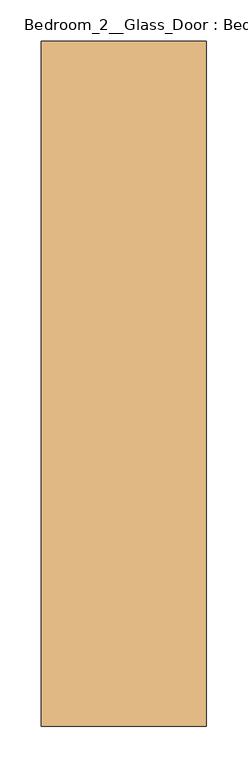
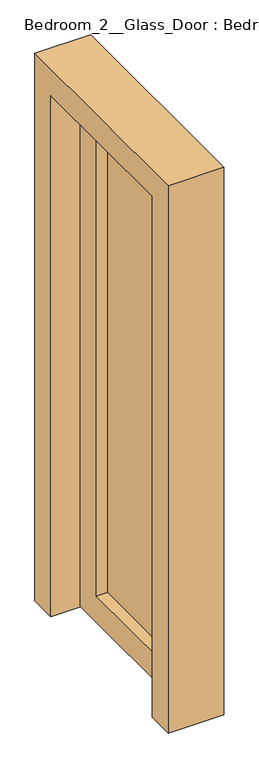
"""IFC4 building model written with IfcOpenShell, lengths in millimetres: door geometry, Bedroom_2__Glass_Door : Bedroom_2__Glass_Door."""

import ifcopenshell
import ifcopenshell.guid

model = None  # the IFC model being written
_history = None  # IfcOwnerHistory: only IFC2X3 demands one
_inside = {}  # id of a spatial element -> (the spatial element, [elements in it])
_under = {}  # id of a project, library or spatial element -> (it, [spatial elements below it])
_declared = {}  # id of a project -> (the project, [libraries it declares])
_typed = {}  # id of a type object -> (the type object, [elements of that type])
_made_of = {}  # id of a material, layer set ... -> (it, [elements and type objects made of it])


def new_model(schema):
    """Start an empty IFC model of exactly this schema.

    Asked for "IFC4X3", IfcOpenShell would pick the latest addendum, in which some entities
    have other attributes; the version numbers below select the first issue.
    IFC2X3 requires an IfcOwnerHistory on every rooted entity: one is made here for all.
    """
    global model, _history
    if schema == "IFC4X3":
        model = ifcopenshell.file(schema_version=(4, 3, 0, 0))
    else:
        model = ifcopenshell.file(schema=schema)
    _inside.clear()
    _under.clear()
    _declared.clear()
    _typed.clear()
    _made_of.clear()
    _history = None
    if model.schema == "IFC2X3":
        org = make("IfcOrganization", Name="unknown")
        user = make(
            "IfcPersonAndOrganization",
            ThePerson=make("IfcPerson", FamilyName="unknown"),
            TheOrganization=org,
        )
        app = make(
            "IfcApplication",
            ApplicationDeveloper=org,
            Version="unknown",
            ApplicationFullName="unknown",
            ApplicationIdentifier="unknown",
        )
        _history = make(
            "IfcOwnerHistory",
            OwningUser=user,
            OwningApplication=app,
            ChangeAction="ADDED",
            CreationDate=0,
        )
    return model


def make(cls, **values):
    """One entity of the class cls with the attributes given. An attribute that is None is left unset."""
    return model.create_entity(
        cls, **{name: value for name, value in values.items() if value is not None}
    )


def rooted(cls, **values):
    """An entity with a GlobalId (a new one), such as an element, a storey or a relation."""
    return make(cls, GlobalId=ifcopenshell.guid.new(), OwnerHistory=_history, **values)


def si_unit(unit_type, name, prefix=None):
    """IfcSIUnit, for example si_unit("LENGTHUNIT", "METRE", prefix="MILLI")."""
    return make("IfcSIUnit", UnitType=unit_type, Prefix=prefix, Name=name)


def assignment(units):
    """IfcUnitAssignment: the units of a project."""
    return None if units is None else make("IfcUnitAssignment", Units=units)


def point(xyz):
    """IfcCartesianPoint."""
    return None if xyz is None else make("IfcCartesianPoint", Coordinates=xyz)


def direction(xyz):
    """IfcDirection."""
    return None if xyz is None else make("IfcDirection", DirectionRatios=xyz)


def frame(location, z_axis=None, x_axis=None):
    """IfcAxis2Placement3D, a coordinate frame: its origin and axes. An axis left out is left unset."""
    return make(
        "IfcAxis2Placement3D",
        Location=point(location),
        Axis=direction(z_axis),
        RefDirection=direction(x_axis),
    )


def origin():
    """The frame at (0, 0, 0) with its axes left unset."""
    return frame((0.0, 0.0, 0.0))


def place(relative_to, where):
    """IfcLocalPlacement: puts the frame where relative to a parent placement (None: the world)."""
    return make(
        "IfcLocalPlacement", PlacementRelTo=relative_to, RelativePlacement=where
    )


def context(
    kind, dimensions, precision=None, world=None, true_north=None, identifier=None
):
    """IfcGeometricRepresentationContext, for example the 3D "Model" context."""
    return make(
        "IfcGeometricRepresentationContext",
        ContextIdentifier=identifier,
        ContextType=kind,
        CoordinateSpaceDimension=dimensions,
        Precision=precision,
        WorldCoordinateSystem=world,
        TrueNorth=true_north,
    )


def project(units=None, contexts=None):
    """IfcProject with its units and contexts."""
    return rooted(
        "IfcProject",
        Name="project",
        RepresentationContexts=contexts,
        UnitsInContext=assignment(units),
    )


def spatial(cls, under=None, at=None, **own):
    """A site, building, storey or space (cls), placed at a placement, below another one or the project."""
    s = rooted(cls, ObjectPlacement=at, **own)
    if under is not None:
        _under.setdefault(under.id(), (under, []))[1].append(s)
    return s


def polyline(points):
    """IfcPolyline through the points."""
    return make("IfcPolyline", Points=[point(p) for p in points])


def outline(outer, holes=None, kind="AREA"):
    """IfcArbitraryClosedProfileDef: a profile drawn as a closed curve; with holes, ...WithVoids."""
    if holes is None:
        return make("IfcArbitraryClosedProfileDef", ProfileType=kind, OuterCurve=outer)
    return make(
        "IfcArbitraryProfileDefWithVoids",
        ProfileType=kind,
        OuterCurve=outer,
        InnerCurves=holes,
    )


def extrude(swept, where, along, depth):
    """IfcExtrudedAreaSolid: the profile swept, set in the frame where, extruded along a direction by depth."""
    return make(
        "IfcExtrudedAreaSolid",
        SweptArea=swept,
        Position=where,
        ExtrudedDirection=direction(along),
        Depth=depth,
    )


def shape(context_of_items, identifier, shape_type, items):
    """IfcShapeRepresentation: the items that make up one representation, for example the "Body"."""
    return make(
        "IfcShapeRepresentation",
        ContextOfItems=context_of_items,
        RepresentationIdentifier=identifier,
        RepresentationType=shape_type,
        Items=items,
    )


def source(mapping_origin, context_of_items, identifier, shape_type, items):
    """IfcRepresentationMap: a shape defined once, which mapped items show again and again."""
    return make(
        "IfcRepresentationMap",
        MappingOrigin=mapping_origin,
        MappedRepresentation=shape(context_of_items, identifier, shape_type, items),
    )


def transform(
    local_origin,
    x_axis=None,
    y_axis=None,
    z_axis=None,
    scale=None,
    scale2=None,
    scale3=None,
    uniform=True,
):
    """IfcCartesianTransformationOperator3D, or its non-uniform kind. x_axis, y_axis, z_axis: its Axis1, 2, 3."""
    if uniform:
        return make(
            "IfcCartesianTransformationOperator3D",
            Axis1=direction(x_axis),
            Axis2=direction(y_axis),
            LocalOrigin=point(local_origin),
            Scale=scale,
            Axis3=direction(z_axis),
        )
    return make(
        "IfcCartesianTransformationOperator3DnonUniform",
        Axis1=direction(x_axis),
        Axis2=direction(y_axis),
        LocalOrigin=point(local_origin),
        Scale=scale,
        Axis3=direction(z_axis),
        Scale2=scale2,
        Scale3=scale3,
    )


def mapped(mapping_source, mapping_target):
    """IfcMappedItem: shows the shape of a source again, moved by a transform."""
    return make(
        "IfcMappedItem", MappingSource=mapping_source, MappingTarget=mapping_target
    )


def made_of(thing, what):
    """Note that an element or type object is made of a material, layer set ...; save() writes the relation."""
    if what is not None:
        _made_of.setdefault(what.id(), (what, []))[1].append(thing)
    return thing


def element(
    cls,
    number,
    at=None,
    inside=None,
    cuts=None,
    type_object=None,
    material=None,
    context=None,
    identifier="Body",
    shape_type=None,
    held_by="IfcProductDefinitionShape",
    body=None,
    shapes=None,
    **own,
):
    """One element of the class cls, such as IfcWall. Its Tag is "e" and its number.

    at: its placement. inside: the storey or other place that contains it. cuts: it is an
    opening in that element (IfcRelVoidsElement). A single representation is given by context,
    identifier, shape_type and body (its items); several are given by shapes. held_by: the class
    of the entity that holds the representations. save() writes the other relations.
    """
    e = rooted(cls, Tag="e%d" % number, ObjectPlacement=at, **own)
    if body is not None:
        shapes = [shape(context, identifier, shape_type, body)]
    if shapes is not None:
        e.Representation = make(held_by, Representations=shapes)
    if inside is not None:
        _inside.setdefault(inside.id(), (inside, []))[1].append(e)
    if cuts is not None:
        rooted(
            "IfcRelVoidsElement", RelatingBuildingElement=cuts, RelatedOpeningElement=e
        )
    if type_object is not None:
        _typed.setdefault(type_object.id(), (type_object, []))[1].append(e)
    return made_of(e, material)


def aggregate(whole, parts):
    """IfcRelAggregates: a whole, such as a stair, and the parts it consists of."""
    return rooted("IfcRelAggregates", RelatingObject=whole, RelatedObjects=parts)


def save(model, path):
    """Write the relations noted so far, then the file.

    IfcRelAggregates (storeys below a building ...), IfcRelContainedInSpatialStructure (elements
    in a storey), IfcRelDefinesByType, IfcRelAssociatesMaterial and IfcRelDeclares: one each for
    every whole, place, type object, material and project.
    """
    for whole, parts in _under.values():
        aggregate(whole, parts)
    for where, things in _inside.values():
        rooted(
            "IfcRelContainedInSpatialStructure",
            RelatedElements=things,
            RelatingStructure=where,
        )
    for kind, things in _typed.values():
        rooted("IfcRelDefinesByType", RelatedObjects=things, RelatingType=kind)
    for what, things in _made_of.values():
        rooted("IfcRelAssociatesMaterial", RelatedObjects=things, RelatingMaterial=what)
    for by, libraries in _declared.values():
        rooted("IfcRelDeclares", RelatingContext=by, RelatedDefinitions=libraries)
    model.write(path)


def bedroom_2_glass_door_bedroom_2_glass_door_faeb561c(model_context):
    return source(origin(), model_context, "Body", "SweptSolid", [
        extrude(outline(polyline([(4355.0, 8175.0), (4355.0, 8585.0), (4365.0, 8585.0), (4365.0, 8175.0), (4355.0, 8175.0)])), frame((0.0, 0.0, 360.0), z_axis=(0.0, 0.0, 1.0), x_axis=(1.0, 0.0, 0.0)), (0.0, 0.0, 1.0), 1760.0),
        extrude(outline(polyline([(8685.0, 2220.0), (8685.0, 260.0), (8075.0, 260.0), (8075.0, 2220.0), (8685.0, 2220.0)]), holes=[polyline([(8585.0, 360.0), (8585.0, 2120.0), (8175.0, 2120.0), (8175.0, 360.0), (8585.0, 360.0)])]), frame((4315.0, 0.0, 0.0), z_axis=(1.0, 0.0, 0.0), x_axis=(0.0, 1.0, 0.0)), (0.0, 0.0, 1.0), 100.0),
        extrude(outline(polyline([(8795.0, 250.0), (8695.0, 250.0), (8695.0, 2230.0), (8065.0, 2230.0), (8065.0, 250.0), (7965.0, 250.0), (7965.0, 2330.0), (8795.0, 2330.0), (8795.0, 250.0)])), frame((4215.0, 0.0, 0.0), z_axis=(1.0, 0.0, 0.0), x_axis=(0.0, 1.0, 0.0)), (0.0, 0.0, 1.0), 200.0),
    ])


if __name__ == "__main__":
    model = new_model("IFC4")
    model_context = context("Model", 3, world=origin())
    ifc_project = project(units=[si_unit("LENGTHUNIT", "METRE", prefix="MILLI")], contexts=[model_context])
    site = spatial("IfcSite", under=ifc_project)
    building = spatial("IfcBuilding", under=site)
    placement = place(None, origin())
    bedroom_2_glass_door_bedroom_2_glass_door_shape = bedroom_2_glass_door_bedroom_2_glass_door_faeb561c(model_context)
    element("IfcDoor", 1, ObjectType="Bedroom_2__Glass_Door : Bedroom_2__Glass_Door", at=placement, inside=building, context=model_context, shape_type="MappedRepresentation", body=[
        mapped(bedroom_2_glass_door_bedroom_2_glass_door_shape, transform((0.0, 0.0, 0.0), x_axis=(1.0, 0.0, 0.0), y_axis=(0.0, 1.0, 0.0), z_axis=(0.0, 0.0, 1.0))),
    ])
    save(model, "model.ifc")

# Revit data of these elements
# Type "Bedroom_2__Glass_Door : Bedroom_2__Glass_Door"
#   Type Mark = "46"
#   NameOverride = "Bedroom_2__Glass_Door"
# Element 1 (IfcDoor, "Bedroom_2__Glass_Door : Bedroom_2__Glass_Door")
#   Materials on its faces: "IfcSurfaceStyle #392", "IfcSurfaceStyle #398"
# Materials
#   "IfcSurfaceStyle #392": class "Unassigned", colour RGB 204 204 204, transparency 0
#   "IfcSurfaceStyle #398": class "Unassigned", colour RGB 93 183 203, transparency 0.85
